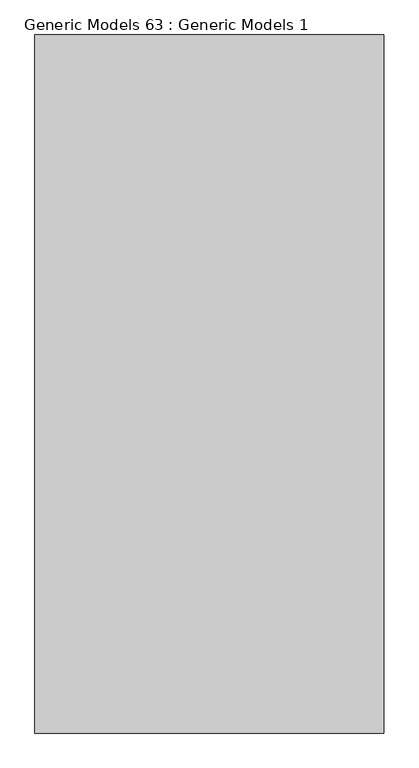
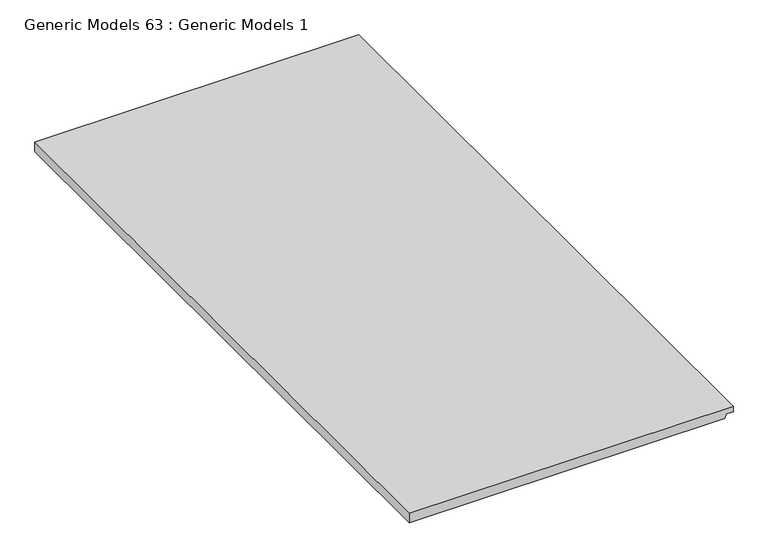
"""IFC4 building model written with IfcOpenShell, lengths in millimetres: proxy geometry, Generic Models 63 : Generic Models 1."""

from ifc_helpers import new_model, si_unit, frame, origin, place, context, project, spatial, polyline, outline, extrude, source, transform, mapped, element, save


def generic_models_63_generic_models_1_24b688b4(model_context):
    return source(origin(), model_context, "Body", "SweptSolid", [
        extrude(outline(polyline([(2253.330428, 51977.6676133), (2253.330428, 51368.0676133), (2234.280428, 51368.0676133), (2234.280428, 51962.0785996), (2242.217928, 51964.9676133), (2242.217928, 51977.6676133), (2253.330428, 51977.6676133)])), frame((0.0, 0.0, 0.0), z_axis=(0.0, 1.0, 0.0), x_axis=(0.0, 0.0, 1.0)), (0.0, 0.0, 1.0), 1219.2),
    ])


if __name__ == "__main__":
    model = new_model("IFC4")
    model_context = context("Model", 3, world=origin())
    ifc_project = project(units=[si_unit("LENGTHUNIT", "METRE", prefix="MILLI")], contexts=[model_context])
    site = spatial("IfcSite", under=ifc_project)
    building = spatial("IfcBuilding", under=site)
    placement = place(None, origin())
    generic_models_63_generic_models_1_shape = generic_models_63_generic_models_1_24b688b4(model_context)
    element("IfcBuildingElementProxy", 1, Name="Generic Models 63 : Generic Models 1", ObjectType="Generic Models 63 : Generic Models 1", at=placement, inside=building, context=model_context, shape_type="MappedRepresentation", body=[
        mapped(generic_models_63_generic_models_1_shape, transform((0.0, 0.0, 0.0), x_axis=(1.0, 0.0, 0.0), y_axis=(0.0, 1.0, 0.0), z_axis=(0.0, 0.0, 1.0))),
    ])
    save(model, "model.ifc")

# Revit data of these elements
# Element 1 (IfcBuildingElementProxy, "Generic Models 63 : Generic Models 1")
#   Materials on its faces: "CEILING AS SCHEDULED"
# Materials
#   "CEILING AS SCHEDULED": class "Generic", colour RGB 255 255 255, transparency 0, Cost = 0
